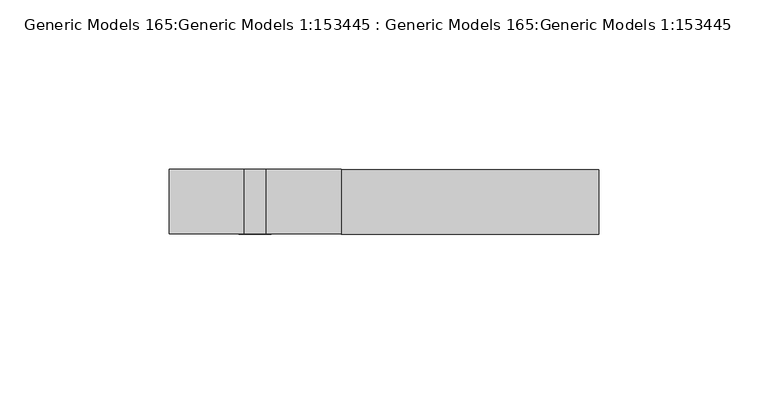
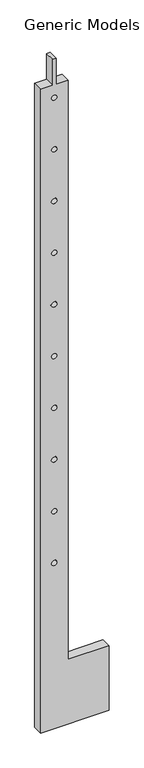
"""IFC4 building model written with IfcOpenShell, lengths in millimetres: proxy geometry, Generic Models 165:Generic Models 1:153445 : Generic Models 165:Generic Models 1:153445."""

from ifc_helpers import new_model, si_unit, point, frame, frame_2d, origin, place, context, project, spatial, polyline, circle_curve, trimmed, segment, composite_curve, outline, extrude, source, transform, mapped, element, save


def generic_models_165_generic_models_1_153445_generic_models_d9ed986d(model_context):
    return source(origin(), model_context, "Body", "SweptSolid", [
        extrude(outline(polyline([(-364.2725126, -10278.9203813), (-364.2725126, -10355.1203813), (773.9649874, -10355.1203813), (773.9649874, -10377.3453813), (824.7649874, -10377.3453813), (824.7649874, -10383.6953813), (773.9649874, -10383.6953813), (773.9649874, -10405.9203813), (-491.2725126, -10405.9203813), (-491.2725126, -10278.9203813), (-364.2725126, -10278.9203813)]), holes=[composite_curve([segment(trimmed(circle_curve(frame_2d((-165.8350126, -10380.5203813)), 4.7625), [point((-165.8350126, -10385.2828813))], [point((-165.8350126, -10375.7578813))], True, "CARTESIAN"), True, "CONTINUOUS"), segment(trimmed(circle_curve(frame_2d((-165.8350126, -10380.5203813)), 4.7625), [point((-165.8350126, -10375.7578813))], [point((-165.8350126, -10385.2828813))], True, "CARTESIAN"), True, "CONTINUOUS")], self_intersect=False), composite_curve([segment(trimmed(circle_curve(frame_2d((-64.2350126, -10380.5203813)), 4.7625), [point((-64.2350126, -10385.2828813))], [point((-64.2350126, -10375.7578813))], True, "CARTESIAN"), True, "CONTINUOUS"), segment(trimmed(circle_curve(frame_2d((-64.2350126, -10380.5203813)), 4.7625), [point((-64.2350126, -10375.7578813))], [point((-64.2350126, -10385.2828813))], True, "CARTESIAN"), True, "CONTINUOUS")], self_intersect=False), composite_curve([segment(trimmed(circle_curve(frame_2d((37.3649874, -10380.5203813)), 4.7625), [point((37.3649874, -10385.2828813))], [point((37.3649874, -10375.7578813))], True, "CARTESIAN"), True, "CONTINUOUS"), segment(trimmed(circle_curve(frame_2d((37.3649874, -10380.5203813)), 4.7625), [point((37.3649874, -10375.7578813))], [point((37.3649874, -10385.2828813))], True, "CARTESIAN"), True, "CONTINUOUS")], self_intersect=False), composite_curve([segment(trimmed(circle_curve(frame_2d((138.9649874, -10380.5203813)), 4.7625), [point((138.9649874, -10385.2828813))], [point((138.9649874, -10375.7578813))], True, "CARTESIAN"), True, "CONTINUOUS"), segment(trimmed(circle_curve(frame_2d((138.9649874, -10380.5203813)), 4.7625), [point((138.9649874, -10375.7578813))], [point((138.9649874, -10385.2828813))], True, "CARTESIAN"), True, "CONTINUOUS")], self_intersect=False), composite_curve([segment(trimmed(circle_curve(frame_2d((240.5649874, -10380.5203813)), 4.7625), [point((240.5649874, -10385.2828813))], [point((240.5649874, -10375.7578813))], True, "CARTESIAN"), True, "CONTINUOUS"), segment(trimmed(circle_curve(frame_2d((240.5649874, -10380.5203813)), 4.7625), [point((240.5649874, -10375.7578813))], [point((240.5649874, -10385.2828813))], True, "CARTESIAN"), True, "CONTINUOUS")], self_intersect=False), composite_curve([segment(trimmed(circle_curve(frame_2d((342.1649874, -10380.5203813)), 4.7625), [point((342.1649874, -10385.2828813))], [point((342.1649874, -10375.7578813))], True, "CARTESIAN"), True, "CONTINUOUS"), segment(trimmed(circle_curve(frame_2d((342.1649874, -10380.5203813)), 4.7625), [point((342.1649874, -10375.7578813))], [point((342.1649874, -10385.2828813))], True, "CARTESIAN"), True, "CONTINUOUS")], self_intersect=False), composite_curve([segment(trimmed(circle_curve(frame_2d((443.7649874, -10380.5203813)), 4.7625), [point((443.7649874, -10385.2828813))], [point((443.7649874, -10375.7578813))], True, "CARTESIAN"), True, "CONTINUOUS"), segment(trimmed(circle_curve(frame_2d((443.7649874, -10380.5203813)), 4.7625), [point((443.7649874, -10375.7578813))], [point((443.7649874, -10385.2828813))], True, "CARTESIAN"), True, "CONTINUOUS")], self_intersect=False), composite_curve([segment(trimmed(circle_curve(frame_2d((545.3649874, -10380.5203813)), 4.7625), [point((545.3649874, -10385.2828813))], [point((545.3649874, -10375.7578813))], True, "CARTESIAN"), True, "CONTINUOUS"), segment(trimmed(circle_curve(frame_2d((545.3649874, -10380.5203813)), 4.7625), [point((545.3649874, -10375.7578813))], [point((545.3649874, -10385.2828813))], True, "CARTESIAN"), True, "CONTINUOUS")], self_intersect=False), composite_curve([segment(trimmed(circle_curve(frame_2d((646.9649874, -10380.5203813)), 4.7625), [point((646.9649874, -10385.2828813))], [point((646.9649874, -10375.7578813))], True, "CARTESIAN"), True, "CONTINUOUS"), segment(trimmed(circle_curve(frame_2d((646.9649874, -10380.5203813)), 4.7625), [point((646.9649874, -10375.7578813))], [point((646.9649874, -10385.2828813))], True, "CARTESIAN"), True, "CONTINUOUS")], self_intersect=False), composite_curve([segment(trimmed(circle_curve(frame_2d((748.5649874, -10380.5203813)), 4.7625), [point((748.5649874, -10385.2828813))], [point((748.5649874, -10375.7578813))], True, "CARTESIAN"), True, "CONTINUOUS"), segment(trimmed(circle_curve(frame_2d((748.5649874, -10380.5203813)), 4.7625), [point((748.5649874, -10375.7578813))], [point((748.5649874, -10385.2828813))], True, "CARTESIAN"), True, "CONTINUOUS")], self_intersect=False)]), frame((0.0, 732.7650592, 0.0), z_axis=(0.0, 1.0, 0.0), x_axis=(0.0, 0.0, 1.0)), (0.0, 0.0, 1.0), 19.05),
    ])


if __name__ == "__main__":
    model = new_model("IFC4")
    model_context = context("Model", 3, world=origin())
    ifc_project = project(units=[si_unit("LENGTHUNIT", "METRE", prefix="MILLI")], contexts=[model_context])
    site = spatial("IfcSite", under=ifc_project)
    building = spatial("IfcBuilding", under=site)
    placement = place(None, origin())
    generic_models_165_generic_models_1_153445_generic_models_shape = generic_models_165_generic_models_1_153445_generic_models_d9ed986d(model_context)
    element("IfcBuildingElementProxy", 1, Name="Generic Models 165:Generic Models 1:153445 : Generic Models 165:Generic Models 1:153445", ObjectType="Generic Models 165:Generic Models 1:153445 : Generic Models 165:Generic Models 1:153445", at=placement, inside=building, context=model_context, shape_type="MappedRepresentation", body=[
        mapped(generic_models_165_generic_models_1_153445_generic_models_shape, transform((0.0, 0.0, 0.0), x_axis=(1.0, 0.0, 0.0), y_axis=(0.0, 1.0, 0.0), z_axis=(0.0, 0.0, 1.0))),
    ])
    save(model, "model.ifc")

# Revit data of these elements
# Type "Generic Models 165:Generic Models 1:153445 : Generic Models 165:Generic Models 1:153445"
#   NameOverride = "Generic Models 165:Generic Models 1:153445"
#   ObjectTypeOverride = "Generic Models 165:Generic Models 1"
#   Reference = "Generic Models 1"
#   Category = "Generic Models"
#   Tag = "153445"
# Element 1 (IfcBuildingElementProxy, "Generic Models 165:Generic Models 1:153445 : Generic Models 165:Generic Models 1:153445")
#   Materials on its faces: "_3/4\" x 1 1/2\" FLAT STOCK PAINTED STEEL POSTS 13787"
# Materials
#   "_3/4\" x 1 1/2\" FLAT STOCK PAINTED STEEL POSTS 13787": class "Unassigned", colour RGB 233 233 233, transparency 0
